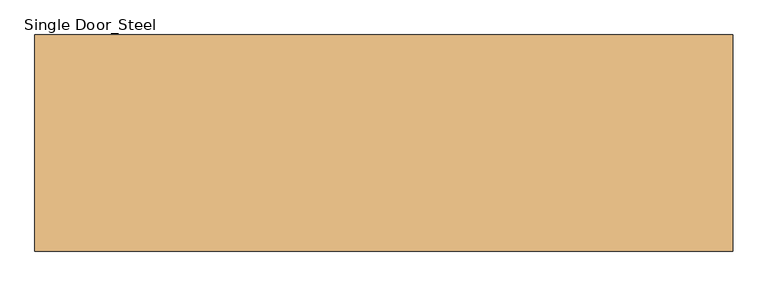
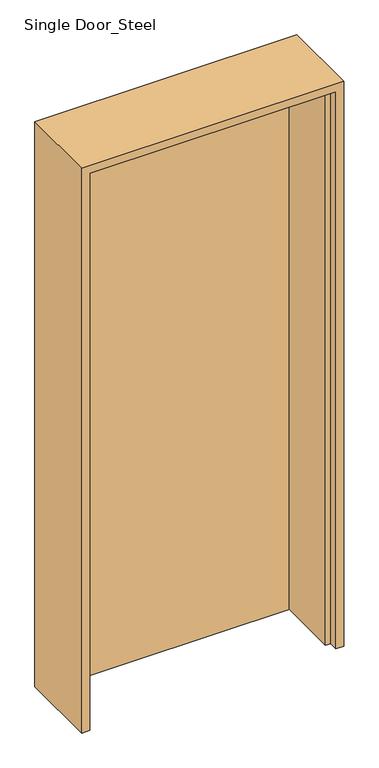
"""IFC4 building model written with IfcOpenShell, lengths in millimetres: door geometry, Single Door_Steel : H_DR_AR_B12_Single Door_Steel_W1000xH2280_FSD1."""

from ifc_helpers import new_model, si_unit, origin, origin_with_axes, place, context, project, spatial, polyline, outline, extrude, faceted_brep, source, transform, mapped, element, save


def single_door_steel_e7c57604(model_context):
    return source(origin(), model_context, "Body", "SolidModel", [
        extrude(outline(polyline([(470.0, 155.0), (470.0, 120.0), (-470.0, 120.0), (-470.0, 155.0), (470.0, 155.0)])), origin_with_axes(), (0.0, 0.0, 1.0), 2250.0),
        faceted_brep([(470.0, 155.0, 0.0), (500.0, 155.0, 0.0), (500.0, -155.0, 0.0), (470.0, -155.0, 0.0), (470.0, -120.0, 0.0), (450.0, -120.0, 0.0), (450.0, 120.0, 0.0), (470.0, 120.0, 0.0), (470.0, 155.0, 2250.0), (-470.0, 155.0, 2250.0), (-470.0, 155.0, 0.0), (-500.0, 155.0, 0.0), (-500.0, 155.0, 2280.0), (500.0, 155.0, 2280.0), (500.0, -155.0, 2280.0), (-500.0, -155.0, 2280.0), (-500.0, -155.0, 0.0), (-470.0, -155.0, 0.0), (-470.0, -155.0, 2250.0), (470.0, -155.0, 2250.0), (470.0, -120.0, 2250.0), (-470.0, -120.0, 2250.0), (-470.0, -120.0, 0.0), (-450.0, -120.0, 0.0), (-450.0, -120.0, 2230.0), (450.0, -120.0, 2230.0), (450.0, 120.0, 2230.0), (-450.0, 120.0, 2230.0), (-450.0, 120.0, 0.0), (-470.0, 120.0, 0.0), (-470.0, 120.0, 2250.0), (470.0, 120.0, 2250.0)], [[[0, 1, 2, 3, 4, 5, 6, 7]], [[1, 0, 8, 9, 10, 11, 12, 13]], [[2, 1, 13, 14]], [[3, 2, 14, 15, 16, 17, 18, 19]], [[4, 3, 19, 20]], [[5, 4, 20, 21, 22, 23, 24, 25]], [[6, 5, 25, 26]], [[7, 6, 26, 27, 28, 29, 30, 31]], [[0, 7, 31, 8]], [[9, 30, 29, 10]], [[10, 29, 28, 23, 22, 17, 16, 11]], [[15, 12, 11, 16]], [[21, 18, 17, 22]], [[27, 24, 23, 28]], [[14, 13, 12, 15]], [[20, 19, 18, 21]], [[26, 25, 24, 27]], [[8, 31, 30, 9]]]),
    ])


if __name__ == "__main__":
    model = new_model("IFC4")
    model_context = context("Model", 3, world=origin())
    ifc_project = project(units=[si_unit("LENGTHUNIT", "METRE", prefix="MILLI")], contexts=[model_context])
    site = spatial("IfcSite", under=ifc_project)
    building = spatial("IfcBuilding", under=site)
    placement = place(None, origin())
    single_door_steel_shape = single_door_steel_e7c57604(model_context)
    element("IfcDoor", 1, ObjectType="Single Door_Steel : H_DR_AR_B12_Single Door_Steel_W1000xH2280_FSD1", at=placement, inside=building, context=model_context, shape_type="MappedRepresentation", body=[
        mapped(single_door_steel_shape, transform((0.0, 0.0, 0.0), x_axis=(1.0, 0.0, 0.0), y_axis=(0.0, 1.0, 0.0), z_axis=(0.0, 0.0, 1.0))),
    ])
    save(model, "model.ifc")

# Revit data of these elements
# Type "Single Door_Steel : H_DR_AR_B12_Single Door_Steel_W1000xH2280_FSD1"
#   Type Mark = "439"
#   Analytic Construction = "<None>"
#   프레임 투영 외부. = 25 mm
#   프레임 투영 내부. = 25 mm
#   프레임 폭 = 75 mm
#   Height = 2280 mm
#   Width = 1000 mm
#   Define Thermal Properties by = 1
#   문 패널 = none
#   문 프레임 = none
#   Function = (empty or 0)
#   Wall Closure = (empty or 0)
